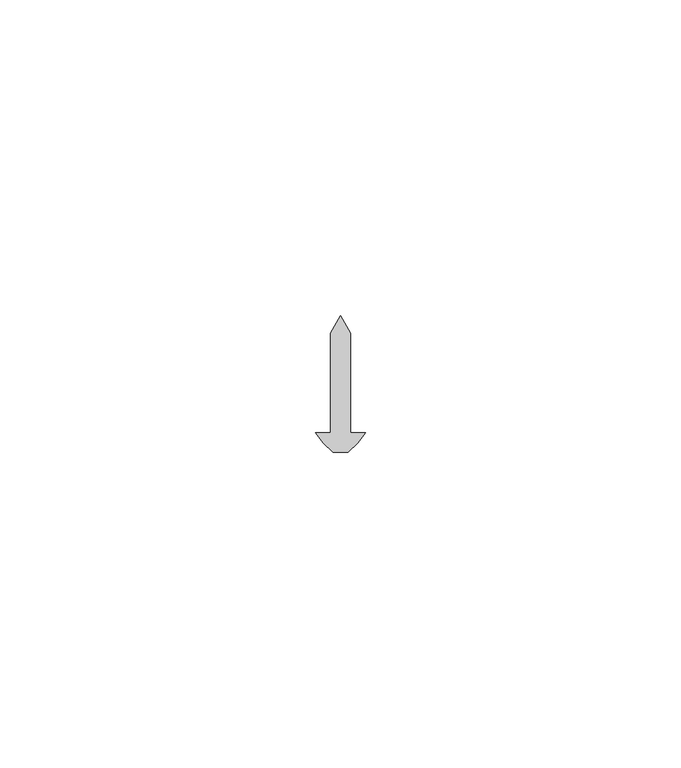
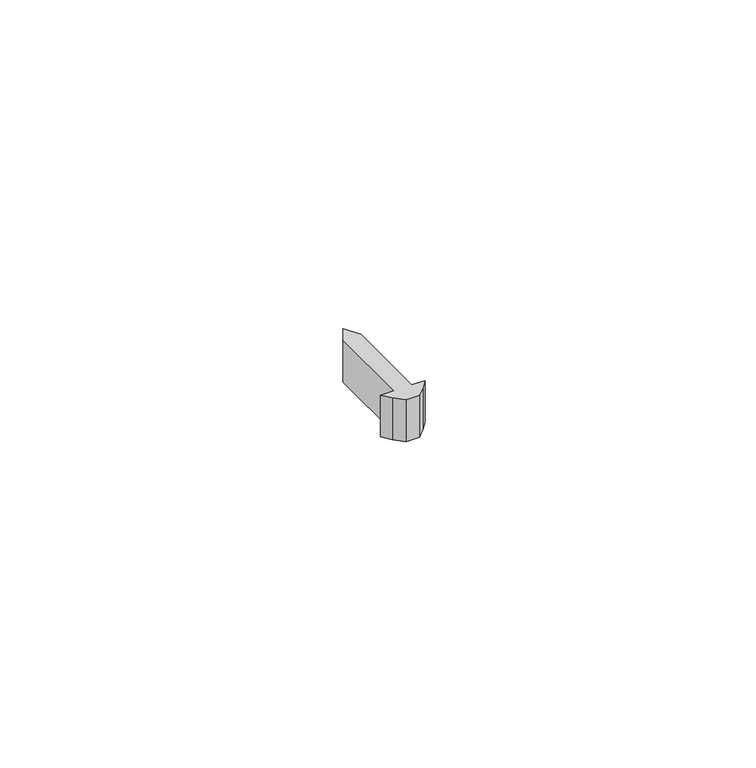
"""IFC4 building model written with IfcOpenShell, lengths in millimetres: proxy geometry, Generic Models 7:Generic Models 1:3:Generic Models 1:3 : Generic Models 7:Generic Models 1:305549:3:Generic Models 1:3:Generic Models 1:3 : Generic Models 7:Generic Models 1:305549:3 : Generic Models 7:Generic Models 1:3:Generic Models 1:3 : Generic Models 7:Generic Models 1:305549:301244:38 : Generic Models 7:Generic Models 1:3:Generic Models 1:3 : Generic Models 7:Generic Models 1:305549:3:Generic Models 1:3:Generic Models 1:3 : Generic Models 7:Generic Models 1:305549:3 : Generic Models 7:Generic Models 1:3:Generic Models 1:3 : Generic Models 7:Generic Models 1:305549:301244:308848."""

import ifcopenshell
import ifcopenshell.guid

model = None  # the IFC model being written
_history = None  # IfcOwnerHistory: only IFC2X3 demands one
_inside = {}  # id of a spatial element -> (the spatial element, [elements in it])
_under = {}  # id of a project, library or spatial element -> (it, [spatial elements below it])
_declared = {}  # id of a project -> (the project, [libraries it declares])
_typed = {}  # id of a type object -> (the type object, [elements of that type])
_made_of = {}  # id of a material, layer set ... -> (it, [elements and type objects made of it])


def new_model(schema):
    """Start an empty IFC model of exactly this schema.

    Asked for "IFC4X3", IfcOpenShell would pick the latest addendum, in which some entities
    have other attributes; the version numbers below select the first issue.
    IFC2X3 requires an IfcOwnerHistory on every rooted entity: one is made here for all.
    """
    global model, _history
    if schema == "IFC4X3":
        model = ifcopenshell.file(schema_version=(4, 3, 0, 0))
    else:
        model = ifcopenshell.file(schema=schema)
    _inside.clear()
    _under.clear()
    _declared.clear()
    _typed.clear()
    _made_of.clear()
    _history = None
    if model.schema == "IFC2X3":
        org = make("IfcOrganization", Name="unknown")
        user = make(
            "IfcPersonAndOrganization",
            ThePerson=make("IfcPerson", FamilyName="unknown"),
            TheOrganization=org,
        )
        app = make(
            "IfcApplication",
            ApplicationDeveloper=org,
            Version="unknown",
            ApplicationFullName="unknown",
            ApplicationIdentifier="unknown",
        )
        _history = make(
            "IfcOwnerHistory",
            OwningUser=user,
            OwningApplication=app,
            ChangeAction="ADDED",
            CreationDate=0,
        )
    return model


def make(cls, **values):
    """One entity of the class cls with the attributes given. An attribute that is None is left unset."""
    return model.create_entity(
        cls, **{name: value for name, value in values.items() if value is not None}
    )


def rooted(cls, **values):
    """An entity with a GlobalId (a new one), such as an element, a storey or a relation."""
    return make(cls, GlobalId=ifcopenshell.guid.new(), OwnerHistory=_history, **values)


def si_unit(unit_type, name, prefix=None):
    """IfcSIUnit, for example si_unit("LENGTHUNIT", "METRE", prefix="MILLI")."""
    return make("IfcSIUnit", UnitType=unit_type, Prefix=prefix, Name=name)


def assignment(units):
    """IfcUnitAssignment: the units of a project."""
    return None if units is None else make("IfcUnitAssignment", Units=units)


def point(xyz):
    """IfcCartesianPoint."""
    return None if xyz is None else make("IfcCartesianPoint", Coordinates=xyz)


def direction(xyz):
    """IfcDirection."""
    return None if xyz is None else make("IfcDirection", DirectionRatios=xyz)


def frame(location, z_axis=None, x_axis=None):
    """IfcAxis2Placement3D, a coordinate frame: its origin and axes. An axis left out is left unset."""
    return make(
        "IfcAxis2Placement3D",
        Location=point(location),
        Axis=direction(z_axis),
        RefDirection=direction(x_axis),
    )


def origin():
    """The frame at (0, 0, 0) with its axes left unset."""
    return frame((0.0, 0.0, 0.0))


def place(relative_to, where):
    """IfcLocalPlacement: puts the frame where relative to a parent placement (None: the world)."""
    return make(
        "IfcLocalPlacement", PlacementRelTo=relative_to, RelativePlacement=where
    )


def context(
    kind, dimensions, precision=None, world=None, true_north=None, identifier=None
):
    """IfcGeometricRepresentationContext, for example the 3D "Model" context."""
    return make(
        "IfcGeometricRepresentationContext",
        ContextIdentifier=identifier,
        ContextType=kind,
        CoordinateSpaceDimension=dimensions,
        Precision=precision,
        WorldCoordinateSystem=world,
        TrueNorth=true_north,
    )


def project(units=None, contexts=None):
    """IfcProject with its units and contexts."""
    return rooted(
        "IfcProject",
        Name="project",
        RepresentationContexts=contexts,
        UnitsInContext=assignment(units),
    )


def spatial(cls, under=None, at=None, **own):
    """A site, building, storey or space (cls), placed at a placement, below another one or the project."""
    s = rooted(cls, ObjectPlacement=at, **own)
    if under is not None:
        _under.setdefault(under.id(), (under, []))[1].append(s)
    return s


def polyline(points):
    """IfcPolyline through the points."""
    return make("IfcPolyline", Points=[point(p) for p in points])


def outline(outer, holes=None, kind="AREA"):
    """IfcArbitraryClosedProfileDef: a profile drawn as a closed curve; with holes, ...WithVoids."""
    if holes is None:
        return make("IfcArbitraryClosedProfileDef", ProfileType=kind, OuterCurve=outer)
    return make(
        "IfcArbitraryProfileDefWithVoids",
        ProfileType=kind,
        OuterCurve=outer,
        InnerCurves=holes,
    )


def extrude(swept, where, along, depth):
    """IfcExtrudedAreaSolid: the profile swept, set in the frame where, extruded along a direction by depth."""
    return make(
        "IfcExtrudedAreaSolid",
        SweptArea=swept,
        Position=where,
        ExtrudedDirection=direction(along),
        Depth=depth,
    )


def shape(context_of_items, identifier, shape_type, items):
    """IfcShapeRepresentation: the items that make up one representation, for example the "Body"."""
    return make(
        "IfcShapeRepresentation",
        ContextOfItems=context_of_items,
        RepresentationIdentifier=identifier,
        RepresentationType=shape_type,
        Items=items,
    )


def source(mapping_origin, context_of_items, identifier, shape_type, items):
    """IfcRepresentationMap: a shape defined once, which mapped items show again and again."""
    return make(
        "IfcRepresentationMap",
        MappingOrigin=mapping_origin,
        MappedRepresentation=shape(context_of_items, identifier, shape_type, items),
    )


def transform(
    local_origin,
    x_axis=None,
    y_axis=None,
    z_axis=None,
    scale=None,
    scale2=None,
    scale3=None,
    uniform=True,
):
    """IfcCartesianTransformationOperator3D, or its non-uniform kind. x_axis, y_axis, z_axis: its Axis1, 2, 3."""
    if uniform:
        return make(
            "IfcCartesianTransformationOperator3D",
            Axis1=direction(x_axis),
            Axis2=direction(y_axis),
            LocalOrigin=point(local_origin),
            Scale=scale,
            Axis3=direction(z_axis),
        )
    return make(
        "IfcCartesianTransformationOperator3DnonUniform",
        Axis1=direction(x_axis),
        Axis2=direction(y_axis),
        LocalOrigin=point(local_origin),
        Scale=scale,
        Axis3=direction(z_axis),
        Scale2=scale2,
        Scale3=scale3,
    )


def mapped(mapping_source, mapping_target):
    """IfcMappedItem: shows the shape of a source again, moved by a transform."""
    return make(
        "IfcMappedItem", MappingSource=mapping_source, MappingTarget=mapping_target
    )


def made_of(thing, what):
    """Note that an element or type object is made of a material, layer set ...; save() writes the relation."""
    if what is not None:
        _made_of.setdefault(what.id(), (what, []))[1].append(thing)
    return thing


def element(
    cls,
    number,
    at=None,
    inside=None,
    cuts=None,
    type_object=None,
    material=None,
    context=None,
    identifier="Body",
    shape_type=None,
    held_by="IfcProductDefinitionShape",
    body=None,
    shapes=None,
    **own,
):
    """One element of the class cls, such as IfcWall. Its Tag is "e" and its number.

    at: its placement. inside: the storey or other place that contains it. cuts: it is an
    opening in that element (IfcRelVoidsElement). A single representation is given by context,
    identifier, shape_type and body (its items); several are given by shapes. held_by: the class
    of the entity that holds the representations. save() writes the other relations.
    """
    e = rooted(cls, Tag="e%d" % number, ObjectPlacement=at, **own)
    if body is not None:
        shapes = [shape(context, identifier, shape_type, body)]
    if shapes is not None:
        e.Representation = make(held_by, Representations=shapes)
    if inside is not None:
        _inside.setdefault(inside.id(), (inside, []))[1].append(e)
    if cuts is not None:
        rooted(
            "IfcRelVoidsElement", RelatingBuildingElement=cuts, RelatedOpeningElement=e
        )
    if type_object is not None:
        _typed.setdefault(type_object.id(), (type_object, []))[1].append(e)
    return made_of(e, material)


def aggregate(whole, parts):
    """IfcRelAggregates: a whole, such as a stair, and the parts it consists of."""
    return rooted("IfcRelAggregates", RelatingObject=whole, RelatedObjects=parts)


def save(model, path):
    """Write the relations noted so far, then the file.

    IfcRelAggregates (storeys below a building ...), IfcRelContainedInSpatialStructure (elements
    in a storey), IfcRelDefinesByType, IfcRelAssociatesMaterial and IfcRelDeclares: one each for
    every whole, place, type object, material and project.
    """
    for whole, parts in _under.values():
        aggregate(whole, parts)
    for where, things in _inside.values():
        rooted(
            "IfcRelContainedInSpatialStructure",
            RelatedElements=things,
            RelatingStructure=where,
        )
    for kind, things in _typed.values():
        rooted("IfcRelDefinesByType", RelatedObjects=things, RelatingType=kind)
    for what, things in _made_of.values():
        rooted("IfcRelAssociatesMaterial", RelatedObjects=things, RelatingMaterial=what)
    for by, libraries in _declared.values():
        rooted("IfcRelDeclares", RelatingContext=by, RelatedDefinitions=libraries)
    model.write(path)


def generic_models_ea78dcf7(model_context):
    return source(origin(), model_context, "Body", "SweptSolid", [
        extrude(outline(polyline([(594346.0992239, -579084.8288841), (594346.0992239, -579069.0196286), (594347.6867239, -579066.2699979), (594349.2742239, -579069.0196286), (594349.2742239, -579084.8288841), (594351.6554739, -579084.8288841), (594350.4372784, -579086.3559421), (594348.8853882, -579087.9078323), (594346.4880597, -579087.9078323), (594344.9361695, -579086.3559421), (594343.7179739, -579084.8288841), (594346.0992239, -579084.8288841)])), frame((0.0, 0.0, 1237.45625), z_axis=(0.0, 0.0, 1.0), x_axis=(1.0, 0.0, 0.0)), (0.0, 0.0, 1.0), 7.9375),
    ])


if __name__ == "__main__":
    model = new_model("IFC4")
    model_context = context("Model", 3, world=origin())
    ifc_project = project(units=[si_unit("LENGTHUNIT", "METRE", prefix="MILLI")], contexts=[model_context])
    site = spatial("IfcSite", under=ifc_project)
    building = spatial("IfcBuilding", under=site)
    placement = place(None, origin())
    generic_models_shape = generic_models_ea78dcf7(model_context)
    element("IfcBuildingElementProxy", 1, Name="Generic Models 7:Generic Models 1:3:Generic Models 1:3 : Generic Models 7:Generic Models 1:305549:3:Generic Models 1:3:Generic Models 1:3 : Generic Models 7:Generic Models 1:305549:3 : Generic Models 7:Generic Models 1:3:Generic Models 1:3 : Generic Models 7:Generic Models 1:305549:301244:38 : Generic Models 7:Generic Models 1:3:Generic Models 1:3 : Generic Models 7:Generic Models 1:305549:3:Generic Models 1:3:Generic Models 1:3 : Generic Models 7:Generic Models 1:305549:3 : Generic Models 7:Generic Models 1:3:Generic Models 1:3 : Generic Models 7:Generic Models 1:305549:301244:308848", ObjectType="Generic Models 7:Generic Models 1:3:Generic Models 1:3 : Generic Models 7:Generic Models 1:305549:3:Generic Models 1:3:Generic Models 1:3 : Generic Models 7:Generic Models 1:305549:3 : Generic Models 7:Generic Models 1:3:Generic Models 1:3 : Generic Models 7:Generic Models 1:305549:301244:38 : Generic Models 7:Generic Models 1:3:Generic Models 1:3 : Generic Models 7:Generic Models 1:305549:3:Generic Models 1:3:Generic Models 1:3 : Generic Models 7:Generic Models 1:305549:3 : Generic Models 7:Generic Models 1:3:Generic Models 1:3 : Generic Models 7:Generic Models 1:305549:301244:308848", at=placement, inside=building, context=model_context, shape_type="MappedRepresentation", body=[
        mapped(generic_models_shape, transform((0.0, 0.0, 0.0), x_axis=(1.0, 0.0, 0.0), y_axis=(0.0, 1.0, 0.0), z_axis=(0.0, 0.0, 1.0))),
    ])
    save(model, "model.ifc")

# Revit data of these elements
# Type "Generic Models 7:Generic Models 1:3:Generic Models 1:3 : Generic Models 7:Generic Models 1:305549:3:Generic Models 1:3:Generic Models 1:3 : Generic Models 7:Generic Models 1:305549:3 : Generic Models 7:Generic Models 1:3:Generic Models 1:3 : Generic Models 7:Generic Models 1:305549:301244:38 : Generic Models 7:Generic Models 1:3:Generic Models 1:3 : Generic Models 7:Generic Models 1:305549:3:Generic Models 1:3:Generic Models 1:3 : Generic Models 7:Generic Models 1:305549:3 : Generic Models 7:Generic Models 1:3:Generic Models 1:3 : Generic Models 7:Generic Models 1:305549:301244:308848"
#   NameOverride = "Generic Models 7:Generic Models 1:3:Generic Models 1:3 : Generic Models 7:Generic Models 1:305549:3:Generic Models 1:3:Generic Models 1:3 : Generic Models 7:Generic Models 1:305549:3 : Generic Models 7:Generic Models 1:3:Generic Models 1:3 : Generic Models 7:Generic Models 1:305549:301244:308848"
#   ObjectTypeOverride = "Generic Models 1:3:Generic Models 1:3 : Generic Models 7:Generic Models 1:305549:3 : Generic Models 7:Generic Models 1:3:Generic Models 1:3 : Generic Models 7:Generic Models 1:305549:301244"
#   Reference = "Generic Models 1"
#   Tag = "308848"
# Element 1 (IfcBuildingElementProxy, "Generic Models 7:Generic Models 1:3:Generic Models 1:3 : Generic Models 7:Generic Models 1:305549:3:Generic Models 1:3:Generic Models 1:3 : Generic Models 7:Generic Models 1:305549:3 : Generic Models 7:Generic Models 1:3:Generic Models 1:3 : Generic Models 7:Generic Models 1:305549:301244:38 : Generic Models 7:Generic Models 1:3:Generic Models 1:3 : Generic Models 7:Generic Models 1:305549:3:Generic Models 1:3:Generic Models 1:3 : Generic Models 7:Generic Models 1:305549:3 : Generic Models 7:Generic Models 1:3:Generic Models 1:3 : Generic Models 7:Generic Models 1:305549:301244:308848")
#   Materials on its faces: "FASTENERS (T.B.D)"
# Materials
#   "FASTENERS (T.B.D)": class "Generic", colour RGB 120 120 120, transparency 0, Cost = 0
